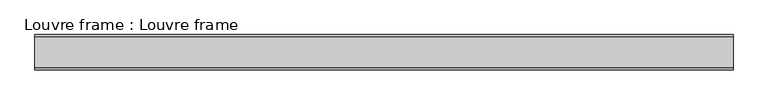
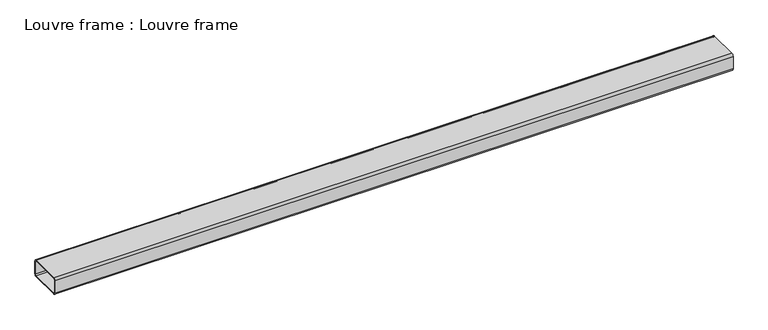
"""IFC4 building model written with IfcOpenShell, lengths in millimetres: proxy geometry, Louvre frame : Louvre frame."""

from ifc_helpers import new_model, si_unit, point, frame, frame_2d, origin, place, context, project, spatial, polyline, circle_curve, trimmed, segment, composite_curve, outline, extrude, source, transform, mapped, element, save


def louvre_frame_louvre_frame_dedd44c9(model_context):
    return source(origin(), model_context, "Body", "SweptSolid", [
        extrude(outline(composite_curve([segment(trimmed(circle_curve(frame_2d((9795.5719584, 39482.0859375)), 6.35), [point((9795.5719584, 39475.7359375))], [point((9789.2219584, 39482.0859375))], False, "CARTESIAN"), True, "CONTINUOUS"), segment(polyline([(9789.2219584, 39482.0859375), (9789.2219584, 39520.1859375)]), True, "CONTINUOUS"), segment(trimmed(circle_curve(frame_2d((9795.5719584, 39520.1859375)), 6.35), [point((9789.2219584, 39520.1859375))], [point((9795.5719584, 39526.5359375))], False, "CARTESIAN"), True, "CONTINUOUS"), segment(polyline([(9795.5719584, 39526.5359375), (9884.4719584, 39526.5359375)]), True, "CONTINUOUS"), segment(trimmed(circle_curve(frame_2d((9884.4719584, 39520.1859375)), 6.35), [point((9884.4719584, 39526.5359375))], [point((9890.8219584, 39520.1859375))], False, "CARTESIAN"), True, "CONTINUOUS"), segment(polyline([(9890.8219584, 39520.1859375), (9890.8219584, 39482.0859375)]), True, "CONTINUOUS"), segment(trimmed(circle_curve(frame_2d((9884.4719584, 39482.0859375)), 6.35), [point((9890.8219584, 39482.0859375))], [point((9884.4719584, 39475.7359375))], False, "CARTESIAN"), True, "CONTINUOUS"), segment(polyline([(9884.4719584, 39475.7359375), (9795.5719584, 39475.7359375)]), True, "CONTINUOUS")], self_intersect=False), holes=[composite_curve([segment(polyline([(9887.6519584, 39482.0859375), (9887.6519584, 39520.1859375)]), True, "CONTINUOUS"), segment(trimmed(circle_curve(frame_2d((9884.4719584, 39520.1859375)), 3.18), [point((9887.6519584, 39520.1859375))], [point((9884.4719584, 39523.3659375))], True, "CARTESIAN"), True, "CONTINUOUS"), segment(polyline([(9884.4719584, 39523.3659375), (9795.5719584, 39523.3659375)]), True, "CONTINUOUS"), segment(trimmed(circle_curve(frame_2d((9795.5719584, 39520.1859375)), 3.18), [point((9795.5719584, 39523.3659375))], [point((9792.3919584, 39520.1859375))], True, "CARTESIAN"), True, "CONTINUOUS"), segment(polyline([(9792.3919584, 39520.1859375), (9792.3919584, 39482.0859375)]), True, "CONTINUOUS"), segment(trimmed(circle_curve(frame_2d((9795.5719584, 39482.0859375)), 3.18), [point((9792.3919584, 39482.0859375))], [point((9795.5719584, 39478.9059375))], True, "CARTESIAN"), True, "CONTINUOUS"), segment(polyline([(9795.5719584, 39478.9059375), (9884.4719584, 39478.9059375)]), True, "CONTINUOUS"), segment(trimmed(circle_curve(frame_2d((9884.4719584, 39482.0859375)), 3.18), [point((9884.4719584, 39478.9059375))], [point((9887.6519584, 39482.0859375))], True, "CARTESIAN"), True, "CONTINUOUS")], self_intersect=False)]), frame((3694.2883192, 0.0, 0.0), z_axis=(1.0, 0.0, 0.0), x_axis=(0.0, 1.0, 0.0)), (0.0, 0.0, 1.0), 2000.0),
    ])


if __name__ == "__main__":
    model = new_model("IFC4")
    model_context = context("Model", 3, world=origin())
    ifc_project = project(units=[si_unit("LENGTHUNIT", "METRE", prefix="MILLI")], contexts=[model_context])
    site = spatial("IfcSite", under=ifc_project)
    building = spatial("IfcBuilding", under=site)
    placement = place(None, origin())
    louvre_frame_louvre_frame_shape = louvre_frame_louvre_frame_dedd44c9(model_context)
    element("IfcBuildingElementProxy", 1, Name="Louvre frame : Louvre frame", ObjectType="Louvre frame : Louvre frame", at=placement, inside=building, context=model_context, shape_type="MappedRepresentation", body=[
        mapped(louvre_frame_louvre_frame_shape, transform((0.0, 0.0, 0.0), x_axis=(1.0, 0.0, 0.0), y_axis=(0.0, 1.0, 0.0), z_axis=(0.0, 0.0, 1.0))),
    ])
    save(model, "model.ifc")

# Revit data of these elements
# Type "Louvre frame : Louvre frame"
#   NameOverride = "Louvre frame"
# Element 1 (IfcBuildingElementProxy, "Louvre frame : Louvre frame")
#   Materials on its faces: "ALUMINIUM LOUVER - TBD"
# Materials
#   "ALUMINIUM LOUVER - TBD": class "Unassigned", colour RGB 92 107 122, transparency 0, Cost = 0
